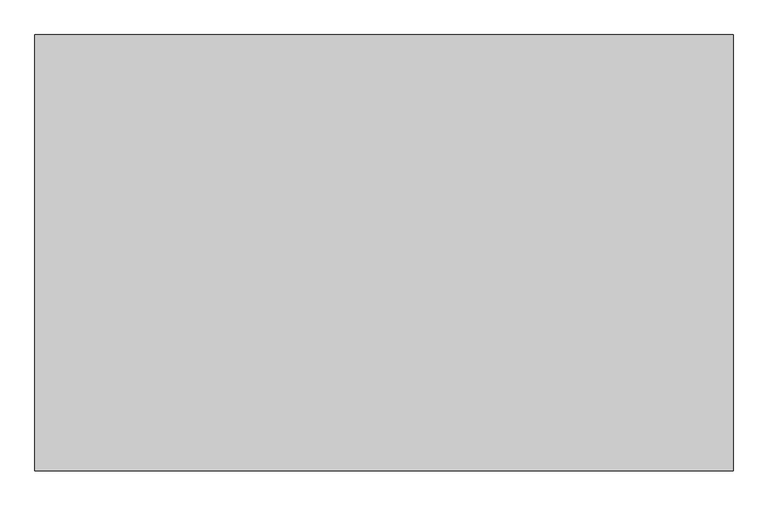
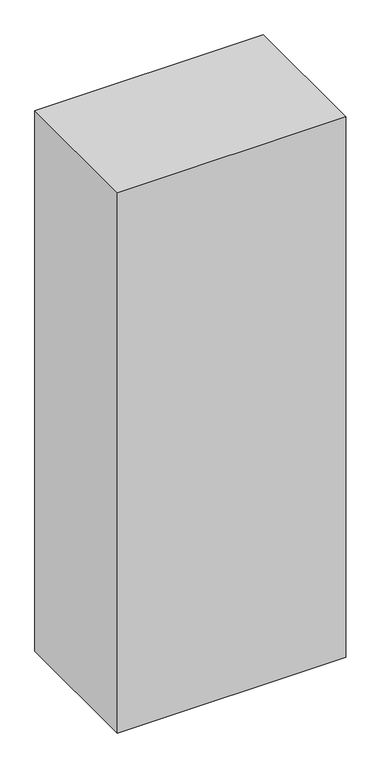
"""IFC4 building model written with IfcOpenShell, lengths in millimetres: proxy geometry, Space Planning Box_hec : Space Planning Box_hec."""

import ifcopenshell
import ifcopenshell.guid

model = None  # the IFC model being written
_history = None  # IfcOwnerHistory: only IFC2X3 demands one
_inside = {}  # id of a spatial element -> (the spatial element, [elements in it])
_under = {}  # id of a project, library or spatial element -> (it, [spatial elements below it])
_declared = {}  # id of a project -> (the project, [libraries it declares])
_typed = {}  # id of a type object -> (the type object, [elements of that type])
_made_of = {}  # id of a material, layer set ... -> (it, [elements and type objects made of it])


def new_model(schema):
    """Start an empty IFC model of exactly this schema.

    Asked for "IFC4X3", IfcOpenShell would pick the latest addendum, in which some entities
    have other attributes; the version numbers below select the first issue.
    IFC2X3 requires an IfcOwnerHistory on every rooted entity: one is made here for all.
    """
    global model, _history
    if schema == "IFC4X3":
        model = ifcopenshell.file(schema_version=(4, 3, 0, 0))
    else:
        model = ifcopenshell.file(schema=schema)
    _inside.clear()
    _under.clear()
    _declared.clear()
    _typed.clear()
    _made_of.clear()
    _history = None
    if model.schema == "IFC2X3":
        org = make("IfcOrganization", Name="unknown")
        user = make(
            "IfcPersonAndOrganization",
            ThePerson=make("IfcPerson", FamilyName="unknown"),
            TheOrganization=org,
        )
        app = make(
            "IfcApplication",
            ApplicationDeveloper=org,
            Version="unknown",
            ApplicationFullName="unknown",
            ApplicationIdentifier="unknown",
        )
        _history = make(
            "IfcOwnerHistory",
            OwningUser=user,
            OwningApplication=app,
            ChangeAction="ADDED",
            CreationDate=0,
        )
    return model


def make(cls, **values):
    """One entity of the class cls with the attributes given. An attribute that is None is left unset."""
    return model.create_entity(
        cls, **{name: value for name, value in values.items() if value is not None}
    )


def rooted(cls, **values):
    """An entity with a GlobalId (a new one), such as an element, a storey or a relation."""
    return make(cls, GlobalId=ifcopenshell.guid.new(), OwnerHistory=_history, **values)


def si_unit(unit_type, name, prefix=None):
    """IfcSIUnit, for example si_unit("LENGTHUNIT", "METRE", prefix="MILLI")."""
    return make("IfcSIUnit", UnitType=unit_type, Prefix=prefix, Name=name)


def assignment(units):
    """IfcUnitAssignment: the units of a project."""
    return None if units is None else make("IfcUnitAssignment", Units=units)


def point(xyz):
    """IfcCartesianPoint."""
    return None if xyz is None else make("IfcCartesianPoint", Coordinates=xyz)


def direction(xyz):
    """IfcDirection."""
    return None if xyz is None else make("IfcDirection", DirectionRatios=xyz)


def frame(location, z_axis=None, x_axis=None):
    """IfcAxis2Placement3D, a coordinate frame: its origin and axes. An axis left out is left unset."""
    return make(
        "IfcAxis2Placement3D",
        Location=point(location),
        Axis=direction(z_axis),
        RefDirection=direction(x_axis),
    )


def origin():
    """The frame at (0, 0, 0) with its axes left unset."""
    return frame((0.0, 0.0, 0.0))


def origin_with_axes():
    """The frame at (0, 0, 0) with the z axis (0, 0, 1) and the x axis (1, 0, 0) written out."""
    return frame((0.0, 0.0, 0.0), z_axis=(0.0, 0.0, 1.0), x_axis=(1.0, 0.0, 0.0))


def place(relative_to, where):
    """IfcLocalPlacement: puts the frame where relative to a parent placement (None: the world)."""
    return make(
        "IfcLocalPlacement", PlacementRelTo=relative_to, RelativePlacement=where
    )


def context(
    kind, dimensions, precision=None, world=None, true_north=None, identifier=None
):
    """IfcGeometricRepresentationContext, for example the 3D "Model" context."""
    return make(
        "IfcGeometricRepresentationContext",
        ContextIdentifier=identifier,
        ContextType=kind,
        CoordinateSpaceDimension=dimensions,
        Precision=precision,
        WorldCoordinateSystem=world,
        TrueNorth=true_north,
    )


def project(units=None, contexts=None):
    """IfcProject with its units and contexts."""
    return rooted(
        "IfcProject",
        Name="project",
        RepresentationContexts=contexts,
        UnitsInContext=assignment(units),
    )


def spatial(cls, under=None, at=None, **own):
    """A site, building, storey or space (cls), placed at a placement, below another one or the project."""
    s = rooted(cls, ObjectPlacement=at, **own)
    if under is not None:
        _under.setdefault(under.id(), (under, []))[1].append(s)
    return s


def polyline(points):
    """IfcPolyline through the points."""
    return make("IfcPolyline", Points=[point(p) for p in points])


def outline(outer, holes=None, kind="AREA"):
    """IfcArbitraryClosedProfileDef: a profile drawn as a closed curve; with holes, ...WithVoids."""
    if holes is None:
        return make("IfcArbitraryClosedProfileDef", ProfileType=kind, OuterCurve=outer)
    return make(
        "IfcArbitraryProfileDefWithVoids",
        ProfileType=kind,
        OuterCurve=outer,
        InnerCurves=holes,
    )


def extrude(swept, where, along, depth):
    """IfcExtrudedAreaSolid: the profile swept, set in the frame where, extruded along a direction by depth."""
    return make(
        "IfcExtrudedAreaSolid",
        SweptArea=swept,
        Position=where,
        ExtrudedDirection=direction(along),
        Depth=depth,
    )


def shape(context_of_items, identifier, shape_type, items):
    """IfcShapeRepresentation: the items that make up one representation, for example the "Body"."""
    return make(
        "IfcShapeRepresentation",
        ContextOfItems=context_of_items,
        RepresentationIdentifier=identifier,
        RepresentationType=shape_type,
        Items=items,
    )


def source(mapping_origin, context_of_items, identifier, shape_type, items):
    """IfcRepresentationMap: a shape defined once, which mapped items show again and again."""
    return make(
        "IfcRepresentationMap",
        MappingOrigin=mapping_origin,
        MappedRepresentation=shape(context_of_items, identifier, shape_type, items),
    )


def transform(
    local_origin,
    x_axis=None,
    y_axis=None,
    z_axis=None,
    scale=None,
    scale2=None,
    scale3=None,
    uniform=True,
):
    """IfcCartesianTransformationOperator3D, or its non-uniform kind. x_axis, y_axis, z_axis: its Axis1, 2, 3."""
    if uniform:
        return make(
            "IfcCartesianTransformationOperator3D",
            Axis1=direction(x_axis),
            Axis2=direction(y_axis),
            LocalOrigin=point(local_origin),
            Scale=scale,
            Axis3=direction(z_axis),
        )
    return make(
        "IfcCartesianTransformationOperator3DnonUniform",
        Axis1=direction(x_axis),
        Axis2=direction(y_axis),
        LocalOrigin=point(local_origin),
        Scale=scale,
        Axis3=direction(z_axis),
        Scale2=scale2,
        Scale3=scale3,
    )


def mapped(mapping_source, mapping_target):
    """IfcMappedItem: shows the shape of a source again, moved by a transform."""
    return make(
        "IfcMappedItem", MappingSource=mapping_source, MappingTarget=mapping_target
    )


def made_of(thing, what):
    """Note that an element or type object is made of a material, layer set ...; save() writes the relation."""
    if what is not None:
        _made_of.setdefault(what.id(), (what, []))[1].append(thing)
    return thing


def element(
    cls,
    number,
    at=None,
    inside=None,
    cuts=None,
    type_object=None,
    material=None,
    context=None,
    identifier="Body",
    shape_type=None,
    held_by="IfcProductDefinitionShape",
    body=None,
    shapes=None,
    **own,
):
    """One element of the class cls, such as IfcWall. Its Tag is "e" and its number.

    at: its placement. inside: the storey or other place that contains it. cuts: it is an
    opening in that element (IfcRelVoidsElement). A single representation is given by context,
    identifier, shape_type and body (its items); several are given by shapes. held_by: the class
    of the entity that holds the representations. save() writes the other relations.
    """
    e = rooted(cls, Tag="e%d" % number, ObjectPlacement=at, **own)
    if body is not None:
        shapes = [shape(context, identifier, shape_type, body)]
    if shapes is not None:
        e.Representation = make(held_by, Representations=shapes)
    if inside is not None:
        _inside.setdefault(inside.id(), (inside, []))[1].append(e)
    if cuts is not None:
        rooted(
            "IfcRelVoidsElement", RelatingBuildingElement=cuts, RelatedOpeningElement=e
        )
    if type_object is not None:
        _typed.setdefault(type_object.id(), (type_object, []))[1].append(e)
    return made_of(e, material)


def aggregate(whole, parts):
    """IfcRelAggregates: a whole, such as a stair, and the parts it consists of."""
    return rooted("IfcRelAggregates", RelatingObject=whole, RelatedObjects=parts)


def save(model, path):
    """Write the relations noted so far, then the file.

    IfcRelAggregates (storeys below a building ...), IfcRelContainedInSpatialStructure (elements
    in a storey), IfcRelDefinesByType, IfcRelAssociatesMaterial and IfcRelDeclares: one each for
    every whole, place, type object, material and project.
    """
    for whole, parts in _under.values():
        aggregate(whole, parts)
    for where, things in _inside.values():
        rooted(
            "IfcRelContainedInSpatialStructure",
            RelatedElements=things,
            RelatingStructure=where,
        )
    for kind, things in _typed.values():
        rooted("IfcRelDefinesByType", RelatedObjects=things, RelatingType=kind)
    for what, things in _made_of.values():
        rooted("IfcRelAssociatesMaterial", RelatedObjects=things, RelatingMaterial=what)
    for by, libraries in _declared.values():
        rooted("IfcRelDeclares", RelatingContext=by, RelatedDefinitions=libraries)
    model.write(path)


def generic_models_7a053eeb(model_context):
    return source(origin(), model_context, "Body", "SweptSolid", [
        extrude(outline(polyline([(1200.0, 750.0), (1200.0, -750.0), (-1200.0, -750.0), (-1200.0, 750.0), (1200.0, 750.0)])), origin_with_axes(), (0.0, 0.0, 1.0), 6000.0),
    ])


if __name__ == "__main__":
    model = new_model("IFC4")
    model_context = context("Model", 3, world=origin())
    ifc_project = project(units=[si_unit("LENGTHUNIT", "METRE", prefix="MILLI")], contexts=[model_context])
    site = spatial("IfcSite", under=ifc_project)
    building = spatial("IfcBuilding", under=site)
    placement = place(None, origin())
    generic_models_shape = generic_models_7a053eeb(model_context)
    element("IfcBuildingElementProxy", 1, Name="Space Planning Box_hec : Space Planning Box_hec", ObjectType="Space Planning Box_hec : Space Planning Box_hec", at=placement, inside=building, context=model_context, shape_type="MappedRepresentation", body=[
        mapped(generic_models_shape, transform((0.0, 0.0, 0.0), x_axis=(1.0, 0.0, 0.0), y_axis=(0.0, 1.0, 0.0), z_axis=(0.0, 0.0, 1.0))),
    ])
    save(model, "model.ifc")

# Revit data of these elements
# Type "Space Planning Box_hec : Space Planning Box_hec"
#   Type Comments = "..."
#   Room Name [instance default] = "?"
#   Interior Finish [instance default] = ""
#   Exterior Finish [instance default] = ""
#   Department [instance default] = ""
#   Assembly Code = "..."
#   Width [instance default] = 1524 mm
#   Program Area [instance default] = 0.00 m²
#   Length [instance default] = 1524 mm
#   Height [instance default] = 1524 mm
#   Area [instance default] = 2.32258 m²
#   Fill Color [instance default] = Cyan
#   Default Elevation = 0
# Element 1 (IfcBuildingElementProxy, "Space Planning Box_hec : Space Planning Box_hec")
#   Room Name = "Shower Room (F)"
#   Interior Finish = "IF5"
#   Exterior Finish = "EF1"
#   Department = "AR"
#   Width = 2400 mm
#   Program Area = 31.50 m²
#   Length = 1500 mm
#   Height = 6000 mm
#   Area = 3.60 m²
#   Fill Color = Lavender
#   Materials on its faces: "Lavender"
# Materials
#   "Cyan": class "Generic", colour RGB 0 255 255, transparency 0.2, Cost = 0
#   "Lavender": class "Generic", colour RGB 186 85 211, transparency 0.2, Cost = 0
